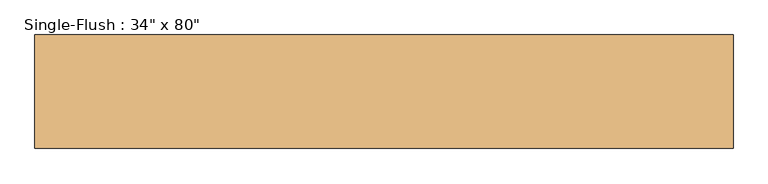
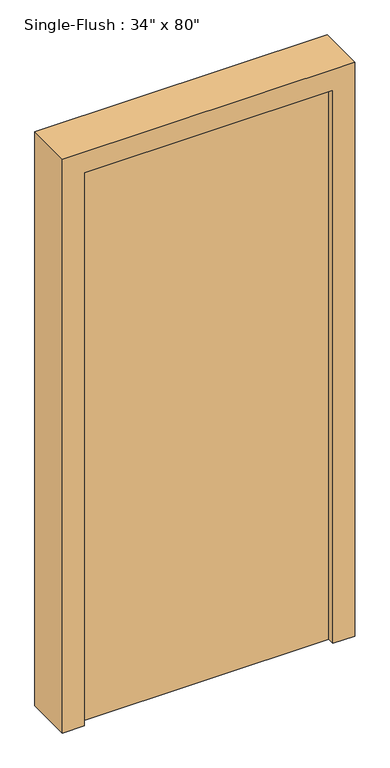
"""IFC4 building model written with IfcOpenShell, lengths in millimetres: door geometry."""

from ifc_helpers import new_model, si_unit, frame, origin, origin_with_axes, place, context, project, spatial, polyline, outline, extrude, source, transform, mapped, element, save


def door_6ce9f8c6(model_context):
    return source(origin(), model_context, "Body", "SweptSolid", [
        extrude(outline(polyline([(2108.2, 508.0), (2108.2, -508.0), (0.0, -508.0), (0.0, -431.8), (2032.0, -431.8), (2032.0, 431.8), (0.0, 431.8), (0.0, 508.0), (2108.2, 508.0)])), frame((0.0, -82.55, 0.0), z_axis=(0.0, 1.0, 0.0), x_axis=(0.0, 0.0, 1.0)), (0.0, 0.0, 1.0), 165.1),
        extrude(outline(polyline([(431.8, -6.35), (431.8, -57.15), (-431.8, -57.15), (-431.8, -6.35), (431.8, -6.35)])), origin_with_axes(), (0.0, 0.0, 1.0), 2032.0),
    ])


if __name__ == "__main__":
    model = new_model("IFC4")
    model_context = context("Model", 3, world=origin())
    ifc_project = project(units=[si_unit("LENGTHUNIT", "METRE", prefix="MILLI")], contexts=[model_context])
    site = spatial("IfcSite", under=ifc_project)
    building = spatial("IfcBuilding", under=site)
    placement = place(None, origin())
    door_shape = door_6ce9f8c6(model_context)
    element("IfcDoor", 1, ObjectType="Single-Flush : 34\" x 80\"", at=placement, inside=building, context=model_context, shape_type="MappedRepresentation", body=[
        mapped(door_shape, transform((0.0, 0.0, 0.0), x_axis=(1.0, 0.0, 0.0), y_axis=(0.0, 1.0, 0.0), z_axis=(0.0, 0.0, 1.0))),
    ])
    save(model, "model.ifc")

# Revit data of these elements
# Type "Single-Flush : 34\" x 80\""
#   Type Mark = "7"
#   OD_DS_Door_Material = "T.B.D."
#   OD_DS_Door_Type = "SWING"
#   OD_DS_Lockset = "PRIVACY LOCK"
#   Assembly Code = "C1020"
#   Analytic Construction = "<None>"
#   Thickness = 0' - 2"
#   RO Offset = 0' - 0 1/4"
#   Height = 6' - 8"
#   Trim Projection Ext = 0' - 1"
#   Trim Projection Int = 0' - 1"
#   Trim Width = 0' - 3"
#   Width = 2' - 10"
#   Door Material = Closet_1
#   Frame Material = Closet_1
#   Function = (empty or 0)
#   Wall Closure = (empty or 0)
# Element 1 (IfcDoor, "Single-Flush : 34\" x 80\"")
#   Materials on its faces: "Closet_1"
# Materials
#   "Closet_1": class "Paint", colour RGB 200 194 183, transparency 0, Cost = 0
